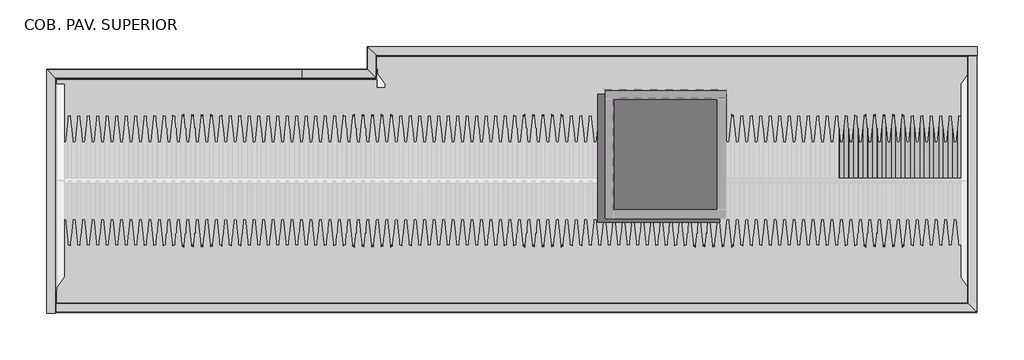
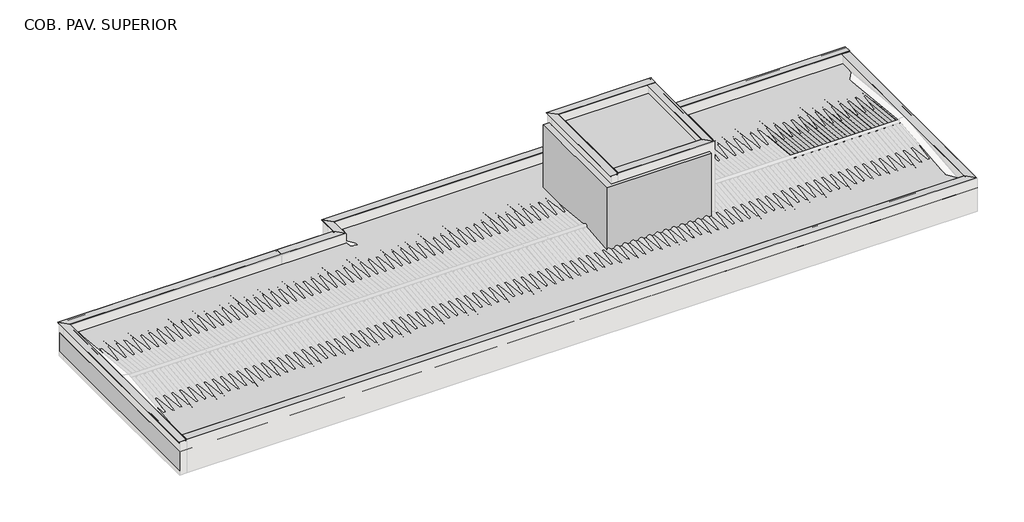
# One storey, part 8 of 8: 25 beams, 7 columns, 4 proxies.
"""IFC4 building model written with IfcOpenShell, lengths in millimetres."""

import ifcopenshell
import ifcopenshell.guid

model = None  # the IFC model being written
_history = None  # IfcOwnerHistory: only IFC2X3 demands one
_inside = {}  # id of a spatial element -> (the spatial element, [elements in it])
_under = {}  # id of a project, library or spatial element -> (it, [spatial elements below it])
_declared = {}  # id of a project -> (the project, [libraries it declares])
_typed = {}  # id of a type object -> (the type object, [elements of that type])
_made_of = {}  # id of a material, layer set ... -> (it, [elements and type objects made of it])


def new_model(schema):
    """Start an empty IFC model of exactly this schema.

    Asked for "IFC4X3", IfcOpenShell would pick the latest addendum, in which some entities
    have other attributes; the version numbers below select the first issue.
    IFC2X3 requires an IfcOwnerHistory on every rooted entity: one is made here for all.
    """
    global model, _history
    if schema == "IFC4X3":
        model = ifcopenshell.file(schema_version=(4, 3, 0, 0))
    else:
        model = ifcopenshell.file(schema=schema)
    _inside.clear()
    _under.clear()
    _declared.clear()
    _typed.clear()
    _made_of.clear()
    _history = None
    if model.schema == "IFC2X3":
        org = make("IfcOrganization", Name="unknown")
        user = make(
            "IfcPersonAndOrganization",
            ThePerson=make("IfcPerson", FamilyName="unknown"),
            TheOrganization=org,
        )
        app = make(
            "IfcApplication",
            ApplicationDeveloper=org,
            Version="unknown",
            ApplicationFullName="unknown",
            ApplicationIdentifier="unknown",
        )
        _history = make(
            "IfcOwnerHistory",
            OwningUser=user,
            OwningApplication=app,
            ChangeAction="ADDED",
            CreationDate=0,
        )
    return model


def make(cls, **values):
    """One entity of the class cls with the attributes given. An attribute that is None is left unset."""
    return model.create_entity(
        cls, **{name: value for name, value in values.items() if value is not None}
    )


def rooted(cls, **values):
    """An entity with a GlobalId (a new one), such as an element, a storey or a relation."""
    return make(cls, GlobalId=ifcopenshell.guid.new(), OwnerHistory=_history, **values)


def si_unit(unit_type, name, prefix=None):
    """IfcSIUnit, for example si_unit("LENGTHUNIT", "METRE", prefix="MILLI")."""
    return make("IfcSIUnit", UnitType=unit_type, Prefix=prefix, Name=name)


def assignment(units):
    """IfcUnitAssignment: the units of a project."""
    return None if units is None else make("IfcUnitAssignment", Units=units)


def point(xyz):
    """IfcCartesianPoint."""
    return None if xyz is None else make("IfcCartesianPoint", Coordinates=xyz)


def direction(xyz):
    """IfcDirection."""
    return None if xyz is None else make("IfcDirection", DirectionRatios=xyz)


def frame(location, z_axis=None, x_axis=None):
    """IfcAxis2Placement3D, a coordinate frame: its origin and axes. An axis left out is left unset."""
    return make(
        "IfcAxis2Placement3D",
        Location=point(location),
        Axis=direction(z_axis),
        RefDirection=direction(x_axis),
    )


def frame_2d(location, x_axis=None):
    """IfcAxis2Placement2D, a coordinate frame in the plane: its origin and x axis."""
    return make(
        "IfcAxis2Placement2D", Location=point(location), RefDirection=direction(x_axis)
    )


def origin():
    """The frame at (0, 0, 0) with its axes left unset."""
    return frame((0.0, 0.0, 0.0))


def place(relative_to, where):
    """IfcLocalPlacement: puts the frame where relative to a parent placement (None: the world)."""
    return make(
        "IfcLocalPlacement", PlacementRelTo=relative_to, RelativePlacement=where
    )


def context(
    kind, dimensions, precision=None, world=None, true_north=None, identifier=None
):
    """IfcGeometricRepresentationContext, for example the 3D "Model" context."""
    return make(
        "IfcGeometricRepresentationContext",
        ContextIdentifier=identifier,
        ContextType=kind,
        CoordinateSpaceDimension=dimensions,
        Precision=precision,
        WorldCoordinateSystem=world,
        TrueNorth=true_north,
    )


def project(units=None, contexts=None):
    """IfcProject with its units and contexts."""
    return rooted(
        "IfcProject",
        Name="project",
        RepresentationContexts=contexts,
        UnitsInContext=assignment(units),
    )


def spatial(cls, under=None, at=None, **own):
    """A site, building, storey or space (cls), placed at a placement, below another one or the project."""
    s = rooted(cls, ObjectPlacement=at, **own)
    if under is not None:
        _under.setdefault(under.id(), (under, []))[1].append(s)
    return s


def polyline(points):
    """IfcPolyline through the points."""
    return make("IfcPolyline", Points=[point(p) for p in points])


def circle_curve(where, radius):
    """IfcCircle in the frame where."""
    return make("IfcCircle", Position=where, Radius=radius)


def trimmed(basis, trim1, trim2, sense, master):
    """IfcTrimmedCurve: the piece of a basis curve between two trims."""
    return make(
        "IfcTrimmedCurve",
        BasisCurve=basis,
        Trim1=trim1,
        Trim2=trim2,
        SenseAgreement=sense,
        MasterRepresentation=master,
    )


def segment(curve, same_sense, transition):
    """IfcCompositeCurveSegment."""
    return make(
        "IfcCompositeCurveSegment",
        Transition=transition,
        SameSense=same_sense,
        ParentCurve=curve,
    )


def composite_curve(segments, self_intersect=None):
    """IfcCompositeCurve: segments joined end to end."""
    return make("IfcCompositeCurve", Segments=segments, SelfIntersect=self_intersect)


def outline(outer, holes=None, kind="AREA"):
    """IfcArbitraryClosedProfileDef: a profile drawn as a closed curve; with holes, ...WithVoids."""
    if holes is None:
        return make("IfcArbitraryClosedProfileDef", ProfileType=kind, OuterCurve=outer)
    return make(
        "IfcArbitraryProfileDefWithVoids",
        ProfileType=kind,
        OuterCurve=outer,
        InnerCurves=holes,
    )


def extrude(swept, where, along, depth):
    """IfcExtrudedAreaSolid: the profile swept, set in the frame where, extruded along a direction by depth."""
    return make(
        "IfcExtrudedAreaSolid",
        SweptArea=swept,
        Position=where,
        ExtrudedDirection=direction(along),
        Depth=depth,
    )


def faces_of(points, faces, orient=None, outer=None):
    """IfcFace entities. A face is a list of loops; a loop is a list of indices into points, from 0.

    orient and outer hold one flag for each loop. By default every Orientation is true, the
    first loop of a face is its IfcFaceOuterBound and the others are IfcFaceBound.
    """
    made = []
    for i, loops in enumerate(faces):
        bounds = []
        for j, loop in enumerate(loops):
            is_outer = j == 0 if outer is None else outer[i][j]
            bounds.append(
                make(
                    "IfcFaceOuterBound" if is_outer else "IfcFaceBound",
                    Bound=make("IfcPolyLoop", Polygon=[points[k] for k in loop]),
                    Orientation=True if orient is None else orient[i][j],
                )
            )
        made.append(make("IfcFace", Bounds=bounds))
    return made


def faceted_brep(points, faces, orient=None, outer=None, voids=None):
    """IfcFacetedBrep: a solid bounded by flat faces; with voids (closed shells), ...WithVoids."""
    shared = [point(p) for p in points]
    hull = make("IfcClosedShell", CfsFaces=faces_of(shared, faces, orient, outer))
    if voids is None:
        return make("IfcFacetedBrep", Outer=hull)
    return make(
        "IfcFacetedBrepWithVoids",
        Outer=hull,
        Voids=[
            make(cls, CfsFaces=faces_of(shared, fs, o, b)) for cls, fs, o, b in voids
        ],
    )


def shape(context_of_items, identifier, shape_type, items):
    """IfcShapeRepresentation: the items that make up one representation, for example the "Body"."""
    return make(
        "IfcShapeRepresentation",
        ContextOfItems=context_of_items,
        RepresentationIdentifier=identifier,
        RepresentationType=shape_type,
        Items=items,
    )


def source(mapping_origin, context_of_items, identifier, shape_type, items):
    """IfcRepresentationMap: a shape defined once, which mapped items show again and again."""
    return make(
        "IfcRepresentationMap",
        MappingOrigin=mapping_origin,
        MappedRepresentation=shape(context_of_items, identifier, shape_type, items),
    )


def transform(
    local_origin,
    x_axis=None,
    y_axis=None,
    z_axis=None,
    scale=None,
    scale2=None,
    scale3=None,
    uniform=True,
):
    """IfcCartesianTransformationOperator3D, or its non-uniform kind. x_axis, y_axis, z_axis: its Axis1, 2, 3."""
    if uniform:
        return make(
            "IfcCartesianTransformationOperator3D",
            Axis1=direction(x_axis),
            Axis2=direction(y_axis),
            LocalOrigin=point(local_origin),
            Scale=scale,
            Axis3=direction(z_axis),
        )
    return make(
        "IfcCartesianTransformationOperator3DnonUniform",
        Axis1=direction(x_axis),
        Axis2=direction(y_axis),
        LocalOrigin=point(local_origin),
        Scale=scale,
        Axis3=direction(z_axis),
        Scale2=scale2,
        Scale3=scale3,
    )


def mapped(mapping_source, mapping_target):
    """IfcMappedItem: shows the shape of a source again, moved by a transform."""
    return make(
        "IfcMappedItem", MappingSource=mapping_source, MappingTarget=mapping_target
    )


def made_of(thing, what):
    """Note that an element or type object is made of a material, layer set ...; save() writes the relation."""
    if what is not None:
        _made_of.setdefault(what.id(), (what, []))[1].append(thing)
    return thing


def element(
    cls,
    number,
    at=None,
    inside=None,
    cuts=None,
    type_object=None,
    material=None,
    context=None,
    identifier="Body",
    shape_type=None,
    held_by="IfcProductDefinitionShape",
    body=None,
    shapes=None,
    **own,
):
    """One element of the class cls, such as IfcWall. Its Tag is "e" and its number.

    at: its placement. inside: the storey or other place that contains it. cuts: it is an
    opening in that element (IfcRelVoidsElement). A single representation is given by context,
    identifier, shape_type and body (its items); several are given by shapes. held_by: the class
    of the entity that holds the representations. save() writes the other relations.
    """
    e = rooted(cls, Tag="e%d" % number, ObjectPlacement=at, **own)
    if body is not None:
        shapes = [shape(context, identifier, shape_type, body)]
    if shapes is not None:
        e.Representation = make(held_by, Representations=shapes)
    if inside is not None:
        _inside.setdefault(inside.id(), (inside, []))[1].append(e)
    if cuts is not None:
        rooted(
            "IfcRelVoidsElement", RelatingBuildingElement=cuts, RelatedOpeningElement=e
        )
    if type_object is not None:
        _typed.setdefault(type_object.id(), (type_object, []))[1].append(e)
    return made_of(e, material)


def aggregate(whole, parts):
    """IfcRelAggregates: a whole, such as a stair, and the parts it consists of."""
    return rooted("IfcRelAggregates", RelatingObject=whole, RelatedObjects=parts)


def save(model, path):
    """Write the relations noted so far, then the file.

    IfcRelAggregates (storeys below a building ...), IfcRelContainedInSpatialStructure (elements
    in a storey), IfcRelDefinesByType, IfcRelAssociatesMaterial and IfcRelDeclares: one each for
    every whole, place, type object, material and project.
    """
    for whole, parts in _under.values():
        aggregate(whole, parts)
    for where, things in _inside.values():
        rooted(
            "IfcRelContainedInSpatialStructure",
            RelatedElements=things,
            RelatingStructure=where,
        )
    for kind, things in _typed.values():
        rooted("IfcRelDefinesByType", RelatedObjects=things, RelatingType=kind)
    for what, things in _made_of.values():
        rooted("IfcRelAssociatesMaterial", RelatedObjects=things, RelatingMaterial=what)
    for by, libraries in _declared.values():
        rooted("IfcRelDeclares", RelatingContext=by, RelatedDefinitions=libraries)
    model.write(path)


def beam_fe4ddbad(model_context):
    return source(origin(), model_context, "Body", "SweptSolid", [
        extrude(outline(polyline([(998.8971968, 30.0), (998.8971968, -30.0), (-998.8971974, -30.0), (-998.8971974, 30.0), (998.8971968, 30.0)])), frame((0.0, 0.0, -60.0), z_axis=(0.0, 0.0, 1.0), x_axis=(1.0, 0.0, 0.0)), (0.0, 0.0, 1.0), 120.0),
    ])


def beam_88f0ebe1(model_context):
    return source(origin(), model_context, "Body", "SweptSolid", [
        extrude(outline(polyline([(136.7503096, 30.0), (136.7503096, -30.0), (-136.7503096, -30.0), (-136.7503096, 30.0), (136.7503096, 30.0)])), frame((0.0, 0.0, -60.0), z_axis=(0.0, 0.0, 1.0), x_axis=(1.0, 0.0, 0.0)), (0.0, 0.0, 1.0), 120.0),
    ])


def beam_c6e4bd39(model_context):
    return source(origin(), model_context, "Body", "SweptSolid", [
        extrude(outline(polyline([(789.5373463, 30.0), (789.5373463, -30.0), (-789.5373463, -30.0), (-789.5373463, 30.0), (789.5373463, 30.0)])), frame((0.0, 0.0, -60.0), z_axis=(0.0, 0.0, 1.0), x_axis=(1.0, 0.0, 0.0)), (0.0, 0.0, 1.0), 120.0),
    ])


def telha_ondulada_fibrocimento_963230a9(model_context):
    return source(origin(), model_context, "Body", "SweptSolid", [
        extrude(outline(composite_curve([segment(trimmed(circle_curve(frame_2d((68.3970135, 71.7939461)), 66.7939461), [point((8.3970135, 42.4437972))], [point((128.3970135, 42.4437972))], True, "CARTESIAN"), True, "CONTINUOUS"), segment(polyline([(128.3970135, 42.4437972), (132.8884385, 40.2467307)]), True, "CONTINUOUS"), segment(trimmed(circle_curve(frame_2d((68.3970135, 71.7939461)), 71.7939461), [point((132.8884385, 40.2467307))], [point((3.9055884, 40.2467307))], False, "CARTESIAN"), True, "CONTINUOUS"), segment(trimmed(circle_curve(frame_2d((-51.6029865, 13.0936483)), 61.7939461), [point((3.9055884, 40.2467307))], [point((-107.1115615, 40.2467307))], True, "CARTESIAN"), True, "CONTINUOUS"), segment(polyline([(-107.1115615, 40.2467307), (-111.6029865, 42.4437972)]), True, "CONTINUOUS"), segment(trimmed(circle_curve(frame_2d((-51.6029865, 13.0936483)), 66.7939461), [point((-111.6029865, 42.4437972))], [point((8.3970135, 42.4437972))], False, "CARTESIAN"), True, "CONTINUOUS")], self_intersect=False)), frame((-362.9289365, 0.0, 0.0), z_axis=(1.0, 0.0, 0.0), x_axis=(0.0, 1.0, 0.0)), (0.0, 0.0, 1.0), 725.8578731),
    ])


def column_6c15bf79(model_context):
    return source(origin(), model_context, "Body", "SweptSolid", [
        extrude(outline(polyline([(30.0, 80.0), (30.0, -80.0), (-30.0, -80.0), (-30.0, 80.0), (30.0, 80.0)])), frame((0.0, 0.0, 6710.0), z_axis=(0.0, 0.0, 1.0), x_axis=(1.0, 0.0, 0.0)), (0.0, 0.0, 1.0), 467.5),
    ])


def column_910cb117(model_context):
    return source(origin(), model_context, "Body", "SweptSolid", [
        extrude(outline(polyline([(30.0, 80.0), (30.0, -80.0), (-30.0, -80.0), (-30.0, 80.0), (30.0, 80.0)])), frame((0.0, 0.0, 6710.0), z_axis=(0.0, 0.0, 1.0), x_axis=(1.0, 0.0, 0.0)), (0.0, 0.0, 1.0), 371.3),
    ])


def column_42eef9f8(model_context):
    return source(origin(), model_context, "Body", "SweptSolid", [
        extrude(outline(polyline([(30.0, 80.0), (30.0, -80.0), (-30.0, -80.0), (-30.0, 80.0), (30.0, 80.0)])), frame((0.0, 0.0, 6710.0), z_axis=(0.0, 0.0, 1.0), x_axis=(1.0, 0.0, 0.0)), (0.0, 0.0, 1.0), 227.1),
    ])


model = new_model("IFC4")

# Units and contexts
model_context = context("Model", 3, world=origin())
ifc_project = project(units=[si_unit("LENGTHUNIT", "METRE", prefix="MILLI")], contexts=[model_context])

# Site, building, storey
site = spatial("IfcSite", under=ifc_project)
building = spatial("IfcBuilding", under=site)
storey = spatial("IfcBuildingStorey", under=building, Name="COB. PAV. SUPERIOR", Elevation=6650.0)

# Beams
placement = place(None, origin())
beam_shape = beam_fe4ddbad(model_context)
element("IfcBeam", 1, ObjectType="Madeira de lei : Berço 6x12cm", at=placement, inside=storey, context=model_context, shape_type="MappedRepresentation", body=[
    mapped(beam_shape, transform((9545.2046801, -7777.6209418, 6680.0), x_axis=(1.0, 0.0, 0.0), y_axis=(0.0, 0.0, -1.0), z_axis=(0.0, 1.0, 0.0))),
])
element("IfcBeam", 2, ObjectType="Madeira de lei : Berço 6x12cm", at=placement, inside=storey, context=model_context, shape_type="MappedRepresentation", body=[
    mapped(beam_shape, transform((7547.4102853, -6365.3711004, 6680.0), x_axis=(1.0, 0.0, 0.0), y_axis=(0.0, 0.0, -1.0), z_axis=(0.0, 1.0, 0.0))),
])
element("IfcBeam", 3, ObjectType="Madeira de lei : Berço 6x12cm", at=placement, inside=storey, context=model_context, shape_type="MappedRepresentation", body=[
    mapped(beam_shape, transform((9545.2046801, -6365.3711004, 6680.0), x_axis=(1.0, 0.0, 0.0), y_axis=(0.0, 0.0, -1.0), z_axis=(0.0, 1.0, 0.0))),
])
element("IfcBeam", 4, ObjectType="Madeira de lei : Berço 6x12cm", at=placement, inside=storey, context=model_context, shape_type="MappedRepresentation", body=[
    mapped(beam_shape, transform((8239.7598386, -4923.3211004, 6680.0), x_axis=(1.0, 0.0, 0.0), y_axis=(0.0, 0.0, -1.0), z_axis=(0.0, 1.0, 0.0))),
])
element("IfcBeam", 5, ObjectType="Madeira de lei : Berço 6x12cm", at=placement, inside=storey, context=model_context, shape_type="MappedRepresentation", body=[
    mapped(beam_shape, transform((6241.9654444, -4923.3211004, 6680.0), x_axis=(1.0, 0.0, 0.0), y_axis=(0.0, 0.0, -1.0), z_axis=(0.0, 1.0, 0.0))),
])
element("IfcBeam", 6, ObjectType="Madeira de lei : Berço 6x12cm", at=placement, inside=storey, context=model_context, shape_type="MappedRepresentation", body=[
    mapped(beam_shape, transform((4244.1710499, -4923.3211004, 6680.0), x_axis=(1.0, 0.0, 0.0), y_axis=(0.0, 0.0, -1.0), z_axis=(0.0, 1.0, 0.0))),
])
beam_2_shape = beam_88f0ebe1(model_context)
element("IfcBeam", 7, ObjectType="Madeira de lei : Berço 6x12cm", at=placement, inside=storey, context=model_context, shape_type="MappedRepresentation", body=[
    mapped(beam_2_shape, transform((10680.8521871, -7777.6209418, 6680.0), x_axis=(1.0, 0.0, 0.0), y_axis=(0.0, 0.0, -1.0), z_axis=(0.0, 1.0, 0.0))),
])
element("IfcBeam", 8, ObjectType="Madeira de lei : Berço 6x12cm", at=placement, inside=storey, context=model_context, shape_type="MappedRepresentation", body=[
    mapped(beam_2_shape, transform((10680.8521871, -6365.3711004, 6680.0), x_axis=(1.0, 0.0, 0.0), y_axis=(0.0, 0.0, -1.0), z_axis=(0.0, 1.0, 0.0))),
])
beam_3_shape = beam_c6e4bd39(model_context)
element("IfcBeam", 9, ObjectType="Madeira de lei : Berço 6x12cm", at=placement, inside=storey, context=model_context, shape_type="MappedRepresentation", body=[
    mapped(beam_3_shape, transform((10028.1943824, -4923.3211004, 6680.0), x_axis=(1.0, 0.0, 0.0), y_axis=(0.0, 0.0, -1.0), z_axis=(0.0, 1.0, 0.0))),
])
element("IfcBeam", 10, ObjectType="Telha Ondulada : Fibrocimento", at=placement, inside=storey, context=model_context, shape_type="SweptSolid", body=[
    extrude(outline(composite_curve([segment(trimmed(circle_curve(frame_2d((-58.7002978, -53.2060539)), 66.7939461), [point((-29.3501489, 6.7939461))], [point((-29.3501489, -113.2060539))], False, "CARTESIAN"), True, "CONTINUOUS"), segment(polyline([(-29.3501489, -113.2060539), (-31.5472154, -108.7146289)]), True, "CONTINUOUS"), segment(trimmed(circle_curve(frame_2d((-58.7002978, -53.2060539)), 61.7939461), [point((-31.5472154, -108.7146289))], [point((-31.5472154, 2.3025211))], True, "CARTESIAN"), True, "CONTINUOUS"), segment(trimmed(circle_curve(frame_2d((0.0, 66.7939461)), 71.7939461), [point((-31.5472154, 2.3025211))], [point((-31.5472154, 131.2853711))], False, "CARTESIAN"), True, "CONTINUOUS"), segment(polyline([(-31.5472154, 131.2853711), (-29.3501489, 126.7939461)]), True, "CONTINUOUS"), segment(trimmed(circle_curve(frame_2d((0.0, 66.7939461)), 66.7939461), [point((-29.3501489, 126.7939461))], [point((-29.3501489, 6.7939461))], True, "CARTESIAN"), True, "CONTINUOUS")], self_intersect=False)), frame((7596.2156257, -4723.1805671, 7106.8215886), z_axis=(0.0, -0.9950371902099893, 0.09950371902099783), x_axis=(0.0, 0.09950371902099783, 0.9950371902099893)), (0.0, 0.0, 1.0), 3060.4439799),
])
element("IfcBeam", 11, ObjectType="Telha Ondulada : Fibrocimento", at=placement, inside=storey, context=model_context, shape_type="SweptSolid", body=[
    extrude(outline(composite_curve([segment(trimmed(circle_curve(frame_2d((-58.7002978, -53.2060539)), 66.7939461), [point((-29.3501489, 6.7939461))], [point((-29.3501489, -113.2060539))], False, "CARTESIAN"), True, "CONTINUOUS"), segment(polyline([(-29.3501489, -113.2060539), (-31.5472154, -108.7146289)]), True, "CONTINUOUS"), segment(trimmed(circle_curve(frame_2d((-58.7002978, -53.2060539)), 61.7939461), [point((-31.5472154, -108.7146289))], [point((-31.5472154, 2.3025211))], True, "CARTESIAN"), True, "CONTINUOUS"), segment(trimmed(circle_curve(frame_2d((0.0, 66.7939461)), 71.7939461), [point((-31.5472154, 2.3025211))], [point((-31.5472154, 131.2853711))], False, "CARTESIAN"), True, "CONTINUOUS"), segment(polyline([(-31.5472154, 131.2853711), (-29.3501489, 126.7939461)]), True, "CONTINUOUS"), segment(trimmed(circle_curve(frame_2d((0.0, 66.7939461)), 66.7939461), [point((-29.3501489, 126.7939461))], [point((-29.3501489, 6.7939461))], True, "CARTESIAN"), True, "CONTINUOUS")], self_intersect=False)), frame((7840.7156257, -4723.1805671, 7106.8215886), z_axis=(0.0, -0.9950371902099893, 0.09950371902099783), x_axis=(0.0, 0.09950371902099783, 0.9950371902099893)), (0.0, 0.0, 1.0), 3060.4439799),
])
element("IfcBeam", 12, ObjectType="Telha Ondulada : Fibrocimento", at=placement, inside=storey, context=model_context, shape_type="SweptSolid", body=[
    extrude(outline(composite_curve([segment(trimmed(circle_curve(frame_2d((-58.7002978, -53.2060539)), 66.7939461), [point((-29.3501489, 6.7939461))], [point((-29.3501489, -113.2060539))], False, "CARTESIAN"), True, "CONTINUOUS"), segment(polyline([(-29.3501489, -113.2060539), (-31.5472154, -108.7146289)]), True, "CONTINUOUS"), segment(trimmed(circle_curve(frame_2d((-58.7002978, -53.2060539)), 61.7939461), [point((-31.5472154, -108.7146289))], [point((-31.5472154, 2.3025211))], True, "CARTESIAN"), True, "CONTINUOUS"), segment(trimmed(circle_curve(frame_2d((0.0, 66.7939461)), 71.7939461), [point((-31.5472154, 2.3025211))], [point((-31.5472154, 131.2853711))], False, "CARTESIAN"), True, "CONTINUOUS"), segment(polyline([(-31.5472154, 131.2853711), (-29.3501489, 126.7939461)]), True, "CONTINUOUS"), segment(trimmed(circle_curve(frame_2d((0.0, 66.7939461)), 66.7939461), [point((-29.3501489, 126.7939461))], [point((-29.3501489, 6.7939461))], True, "CARTESIAN"), True, "CONTINUOUS")], self_intersect=False)), frame((8085.2156257, -4723.1805671, 7106.8215886), z_axis=(0.0, -0.9950371902099893, 0.09950371902099783), x_axis=(0.0, 0.09950371902099783, 0.9950371902099893)), (0.0, 0.0, 1.0), 3060.4439799),
])
element("IfcBeam", 13, ObjectType="Telha Ondulada : Fibrocimento", at=placement, inside=storey, context=model_context, shape_type="SweptSolid", body=[
    extrude(outline(composite_curve([segment(trimmed(circle_curve(frame_2d((-58.7002978, -53.2060539)), 66.7939461), [point((-29.3501489, 6.7939461))], [point((-29.3501489, -113.2060539))], False, "CARTESIAN"), True, "CONTINUOUS"), segment(polyline([(-29.3501489, -113.2060539), (-31.5472154, -108.7146289)]), True, "CONTINUOUS"), segment(trimmed(circle_curve(frame_2d((-58.7002978, -53.2060539)), 61.7939461), [point((-31.5472154, -108.7146289))], [point((-31.5472154, 2.3025211))], True, "CARTESIAN"), True, "CONTINUOUS"), segment(trimmed(circle_curve(frame_2d((0.0, 66.7939461)), 71.7939461), [point((-31.5472154, 2.3025211))], [point((-31.5472154, 131.2853711))], False, "CARTESIAN"), True, "CONTINUOUS"), segment(polyline([(-31.5472154, 131.2853711), (-29.3501489, 126.7939461)]), True, "CONTINUOUS"), segment(trimmed(circle_curve(frame_2d((0.0, 66.7939461)), 66.7939461), [point((-29.3501489, 126.7939461))], [point((-29.3501489, 6.7939461))], True, "CARTESIAN"), True, "CONTINUOUS")], self_intersect=False)), frame((8329.7156257, -4723.1805671, 7106.8215886), z_axis=(0.0, -0.9950371902099893, 0.09950371902099785), x_axis=(0.0, 0.09950371902099785, 0.9950371902099893)), (0.0, 0.0, 1.0), 3060.4439799),
])
element("IfcBeam", 14, ObjectType="Telha Ondulada : Fibrocimento", at=placement, inside=storey, context=model_context, shape_type="SweptSolid", body=[
    extrude(outline(composite_curve([segment(trimmed(circle_curve(frame_2d((-58.7002978, -53.2060539)), 66.7939461), [point((-29.3501489, 6.7939461))], [point((-29.3501489, -113.2060539))], False, "CARTESIAN"), True, "CONTINUOUS"), segment(polyline([(-29.3501489, -113.2060539), (-31.5472154, -108.7146289)]), True, "CONTINUOUS"), segment(trimmed(circle_curve(frame_2d((-58.7002978, -53.2060539)), 61.7939461), [point((-31.5472154, -108.7146289))], [point((-31.5472154, 2.3025211))], True, "CARTESIAN"), True, "CONTINUOUS"), segment(trimmed(circle_curve(frame_2d((0.0, 66.7939461)), 71.7939461), [point((-31.5472154, 2.3025211))], [point((-31.5472154, 131.2853711))], False, "CARTESIAN"), True, "CONTINUOUS"), segment(polyline([(-31.5472154, 131.2853711), (-29.3501489, 126.7939461)]), True, "CONTINUOUS"), segment(trimmed(circle_curve(frame_2d((0.0, 66.7939461)), 66.7939461), [point((-29.3501489, 126.7939461))], [point((-29.3501489, 6.7939461))], True, "CARTESIAN"), True, "CONTINUOUS")], self_intersect=False)), frame((8574.2156257, -4723.1805671, 7106.8215886), z_axis=(0.0, -0.9950371902099893, 0.0995037190209978), x_axis=(0.0, 0.0995037190209978, 0.9950371902099893)), (0.0, 0.0, 1.0), 3060.4439799),
])
element("IfcBeam", 15, ObjectType="Telha Ondulada : Fibrocimento", at=placement, inside=storey, context=model_context, shape_type="SweptSolid", body=[
    extrude(outline(composite_curve([segment(trimmed(circle_curve(frame_2d((-58.7002978, -53.2060539)), 66.7939461), [point((-29.3501489, 6.7939461))], [point((-29.3501489, -113.2060539))], False, "CARTESIAN"), True, "CONTINUOUS"), segment(polyline([(-29.3501489, -113.2060539), (-31.5472154, -108.7146289)]), True, "CONTINUOUS"), segment(trimmed(circle_curve(frame_2d((-58.7002978, -53.2060539)), 61.7939461), [point((-31.5472154, -108.7146289))], [point((-31.5472154, 2.3025211))], True, "CARTESIAN"), True, "CONTINUOUS"), segment(trimmed(circle_curve(frame_2d((0.0, 66.7939461)), 71.7939461), [point((-31.5472154, 2.3025211))], [point((-31.5472154, 131.2853711))], False, "CARTESIAN"), True, "CONTINUOUS"), segment(polyline([(-31.5472154, 131.2853711), (-29.3501489, 126.7939461)]), True, "CONTINUOUS"), segment(trimmed(circle_curve(frame_2d((0.0, 66.7939461)), 66.7939461), [point((-29.3501489, 126.7939461))], [point((-29.3501489, 6.7939461))], True, "CARTESIAN"), True, "CONTINUOUS")], self_intersect=False)), frame((8818.7156257, -4723.1805671, 7106.8215886), z_axis=(0.0, -0.9950371902099893, 0.0995037190209978), x_axis=(0.0, 0.0995037190209978, 0.9950371902099893)), (0.0, 0.0, 1.0), 3060.4439799),
])
element("IfcBeam", 16, ObjectType="Telha Ondulada : Fibrocimento", at=placement, inside=storey, context=model_context, shape_type="SweptSolid", body=[
    extrude(outline(composite_curve([segment(trimmed(circle_curve(frame_2d((-58.7002978, -53.2060539)), 66.7939461), [point((-29.3501489, 6.7939461))], [point((-29.3501489, -113.2060539))], False, "CARTESIAN"), True, "CONTINUOUS"), segment(polyline([(-29.3501489, -113.2060539), (-31.5472154, -108.7146289)]), True, "CONTINUOUS"), segment(trimmed(circle_curve(frame_2d((-58.7002978, -53.2060539)), 61.7939461), [point((-31.5472154, -108.7146289))], [point((-31.5472154, 2.3025211))], True, "CARTESIAN"), True, "CONTINUOUS"), segment(trimmed(circle_curve(frame_2d((0.0, 66.7939461)), 71.7939461), [point((-31.5472154, 2.3025211))], [point((-31.5472154, 131.2853711))], False, "CARTESIAN"), True, "CONTINUOUS"), segment(polyline([(-31.5472154, 131.2853711), (-29.3501489, 126.7939461)]), True, "CONTINUOUS"), segment(trimmed(circle_curve(frame_2d((0.0, 66.7939461)), 66.7939461), [point((-29.3501489, 126.7939461))], [point((-29.3501489, 6.7939461))], True, "CARTESIAN"), True, "CONTINUOUS")], self_intersect=False)), frame((9063.2156257, -4723.1805671, 7106.8215886), z_axis=(0.0, -0.9950371902099893, 0.0995037190209978), x_axis=(0.0, 0.0995037190209978, 0.9950371902099893)), (0.0, 0.0, 1.0), 3060.4439799),
])
element("IfcBeam", 17, ObjectType="Telha Ondulada : Fibrocimento", at=placement, inside=storey, context=model_context, shape_type="SweptSolid", body=[
    extrude(outline(composite_curve([segment(trimmed(circle_curve(frame_2d((-58.7002978, -53.2060539)), 66.7939461), [point((-29.3501489, 6.7939461))], [point((-29.3501489, -113.2060539))], False, "CARTESIAN"), True, "CONTINUOUS"), segment(polyline([(-29.3501489, -113.2060539), (-31.5472154, -108.7146289)]), True, "CONTINUOUS"), segment(trimmed(circle_curve(frame_2d((-58.7002978, -53.2060539)), 61.7939461), [point((-31.5472154, -108.7146289))], [point((-31.5472154, 2.3025211))], True, "CARTESIAN"), True, "CONTINUOUS"), segment(trimmed(circle_curve(frame_2d((0.0, 66.7939461)), 71.7939461), [point((-31.5472154, 2.3025211))], [point((-31.5472154, 131.2853711))], False, "CARTESIAN"), True, "CONTINUOUS"), segment(polyline([(-31.5472154, 131.2853711), (-29.3501489, 126.7939461)]), True, "CONTINUOUS"), segment(trimmed(circle_curve(frame_2d((0.0, 66.7939461)), 66.7939461), [point((-29.3501489, 126.7939461))], [point((-29.3501489, 6.7939461))], True, "CARTESIAN"), True, "CONTINUOUS")], self_intersect=False)), frame((9307.7156257, -4723.1805671, 7106.8215886), z_axis=(0.0, -0.9950371902099893, 0.0995037190209978), x_axis=(0.0, 0.0995037190209978, 0.9950371902099893)), (0.0, 0.0, 1.0), 3060.4439799),
])
element("IfcBeam", 18, ObjectType="Telha Ondulada : Fibrocimento", at=placement, inside=storey, context=model_context, shape_type="SweptSolid", body=[
    extrude(outline(composite_curve([segment(trimmed(circle_curve(frame_2d((-58.7002978, -53.2060539)), 66.7939461), [point((-29.3501489, 6.7939461))], [point((-29.3501489, -113.2060539))], False, "CARTESIAN"), True, "CONTINUOUS"), segment(polyline([(-29.3501489, -113.2060539), (-31.5472154, -108.7146289)]), True, "CONTINUOUS"), segment(trimmed(circle_curve(frame_2d((-58.7002978, -53.2060539)), 61.7939461), [point((-31.5472154, -108.7146289))], [point((-31.5472154, 2.3025211))], True, "CARTESIAN"), True, "CONTINUOUS"), segment(trimmed(circle_curve(frame_2d((0.0, 66.7939461)), 71.7939461), [point((-31.5472154, 2.3025211))], [point((-31.5472154, 131.2853711))], False, "CARTESIAN"), True, "CONTINUOUS"), segment(polyline([(-31.5472154, 131.2853711), (-29.3501489, 126.7939461)]), True, "CONTINUOUS"), segment(trimmed(circle_curve(frame_2d((0.0, 66.7939461)), 66.7939461), [point((-29.3501489, 126.7939461))], [point((-29.3501489, 6.7939461))], True, "CARTESIAN"), True, "CONTINUOUS")], self_intersect=False)), frame((9552.2156257, -4723.1805671, 7106.8215886), z_axis=(0.0, -0.9950371902099893, 0.0995037190209978), x_axis=(0.0, 0.0995037190209978, 0.9950371902099893)), (0.0, 0.0, 1.0), 3060.4439799),
])
element("IfcBeam", 19, ObjectType="Telha Ondulada : Fibrocimento", at=placement, inside=storey, context=model_context, shape_type="SweptSolid", body=[
    extrude(outline(composite_curve([segment(trimmed(circle_curve(frame_2d((-58.7002978, -53.2060539)), 66.7939461), [point((-29.3501489, 6.7939461))], [point((-29.3501489, -113.2060539))], False, "CARTESIAN"), True, "CONTINUOUS"), segment(polyline([(-29.3501489, -113.2060539), (-31.5472154, -108.7146289)]), True, "CONTINUOUS"), segment(trimmed(circle_curve(frame_2d((-58.7002978, -53.2060539)), 61.7939461), [point((-31.5472154, -108.7146289))], [point((-31.5472154, 2.3025211))], True, "CARTESIAN"), True, "CONTINUOUS"), segment(trimmed(circle_curve(frame_2d((0.0, 66.7939461)), 71.7939461), [point((-31.5472154, 2.3025211))], [point((-31.5472154, 131.2853711))], False, "CARTESIAN"), True, "CONTINUOUS"), segment(polyline([(-31.5472154, 131.2853711), (-29.3501489, 126.7939461)]), True, "CONTINUOUS"), segment(trimmed(circle_curve(frame_2d((0.0, 66.7939461)), 66.7939461), [point((-29.3501489, 126.7939461))], [point((-29.3501489, 6.7939461))], True, "CARTESIAN"), True, "CONTINUOUS")], self_intersect=False)), frame((9796.7156257, -4723.1805671, 7106.8215886), z_axis=(0.0, -0.9950371902099893, 0.0995037190209978), x_axis=(0.0, 0.0995037190209978, 0.9950371902099893)), (0.0, 0.0, 1.0), 3060.4439799),
])
element("IfcBeam", 20, ObjectType="Telha Ondulada : Fibrocimento", at=placement, inside=storey, context=model_context, shape_type="SweptSolid", body=[
    extrude(outline(composite_curve([segment(trimmed(circle_curve(frame_2d((-58.7002978, -53.2060539)), 66.7939461), [point((-29.3501489, 6.7939461))], [point((-29.3501489, -113.2060539))], False, "CARTESIAN"), True, "CONTINUOUS"), segment(polyline([(-29.3501489, -113.2060539), (-31.5472154, -108.7146289)]), True, "CONTINUOUS"), segment(trimmed(circle_curve(frame_2d((-58.7002978, -53.2060539)), 61.7939461), [point((-31.5472154, -108.7146289))], [point((-31.5472154, 2.3025211))], True, "CARTESIAN"), True, "CONTINUOUS"), segment(trimmed(circle_curve(frame_2d((0.0, 66.7939461)), 71.7939461), [point((-31.5472154, 2.3025211))], [point((-31.5472154, 131.2853711))], False, "CARTESIAN"), True, "CONTINUOUS"), segment(polyline([(-31.5472154, 131.2853711), (-29.3501489, 126.7939461)]), True, "CONTINUOUS"), segment(trimmed(circle_curve(frame_2d((0.0, 66.7939461)), 66.7939461), [point((-29.3501489, 126.7939461))], [point((-29.3501489, 6.7939461))], True, "CARTESIAN"), True, "CONTINUOUS")], self_intersect=False)), frame((10041.2156257, -4723.1805671, 7106.8215886), z_axis=(0.0, -0.9950371902099893, 0.0995037190209978), x_axis=(0.0, 0.0995037190209978, 0.9950371902099893)), (0.0, 0.0, 1.0), 3060.4439799),
])
element("IfcBeam", 21, ObjectType="Telha Ondulada : Fibrocimento", at=placement, inside=storey, context=model_context, shape_type="SweptSolid", body=[
    extrude(outline(composite_curve([segment(trimmed(circle_curve(frame_2d((-58.7002978, -53.2060539)), 66.7939461), [point((-29.3501489, 6.7939461))], [point((-29.3501489, -113.2060539))], False, "CARTESIAN"), True, "CONTINUOUS"), segment(polyline([(-29.3501489, -113.2060539), (-31.5472154, -108.7146289)]), True, "CONTINUOUS"), segment(trimmed(circle_curve(frame_2d((-58.7002978, -53.2060539)), 61.7939461), [point((-31.5472154, -108.7146289))], [point((-31.5472154, 2.3025211))], True, "CARTESIAN"), True, "CONTINUOUS"), segment(trimmed(circle_curve(frame_2d((0.0, 66.7939461)), 71.7939461), [point((-31.5472154, 2.3025211))], [point((-31.5472154, 131.2853711))], False, "CARTESIAN"), True, "CONTINUOUS"), segment(polyline([(-31.5472154, 131.2853711), (-29.3501489, 126.7939461)]), True, "CONTINUOUS"), segment(trimmed(circle_curve(frame_2d((0.0, 66.7939461)), 66.7939461), [point((-29.3501489, 126.7939461))], [point((-29.3501489, 6.7939461))], True, "CARTESIAN"), True, "CONTINUOUS")], self_intersect=False)), frame((10285.7156257, -4723.1805671, 7106.8215886), z_axis=(0.0, -0.9950371902099893, 0.0995037190209978), x_axis=(0.0, 0.0995037190209978, 0.9950371902099893)), (0.0, 0.0, 1.0), 3060.4439799),
])
element("IfcBeam", 22, ObjectType="Telha Ondulada : Fibrocimento", at=placement, inside=storey, context=model_context, shape_type="SweptSolid", body=[
    extrude(outline(composite_curve([segment(trimmed(circle_curve(frame_2d((-58.7002978, -53.2060539)), 66.7939461), [point((-29.3501489, 6.7939461))], [point((-29.3501489, -113.2060539))], False, "CARTESIAN"), True, "CONTINUOUS"), segment(polyline([(-29.3501489, -113.2060539), (-31.5472154, -108.7146289)]), True, "CONTINUOUS"), segment(trimmed(circle_curve(frame_2d((-58.7002978, -53.2060539)), 61.7939461), [point((-31.5472154, -108.7146289))], [point((-31.5472154, 2.3025211))], True, "CARTESIAN"), True, "CONTINUOUS"), segment(trimmed(circle_curve(frame_2d((0.0, 66.7939461)), 71.7939461), [point((-31.5472154, 2.3025211))], [point((-31.5472154, 131.2853711))], False, "CARTESIAN"), True, "CONTINUOUS"), segment(polyline([(-31.5472154, 131.2853711), (-29.3501489, 126.7939461)]), True, "CONTINUOUS"), segment(trimmed(circle_curve(frame_2d((0.0, 66.7939461)), 66.7939461), [point((-29.3501489, 126.7939461))], [point((-29.3501489, 6.7939461))], True, "CARTESIAN"), True, "CONTINUOUS")], self_intersect=False)), frame((10530.2156257, -4723.1805671, 7106.8215886), z_axis=(0.0, -0.9950371902099893, 0.0995037190209978), x_axis=(0.0, 0.0995037190209978, 0.9950371902099893)), (0.0, 0.0, 1.0), 3060.4439799),
])
element("IfcBeam", 23, ObjectType="Telha Ondulada : Fibrocimento", at=placement, inside=storey, context=model_context, shape_type="SweptSolid", body=[
    extrude(outline(composite_curve([segment(trimmed(circle_curve(frame_2d((-58.7002978, -53.2060539)), 66.7939461), [point((-29.3501489, 6.7939461))], [point((-29.3501489, -113.2060539))], False, "CARTESIAN"), True, "CONTINUOUS"), segment(polyline([(-29.3501489, -113.2060539), (-31.5472154, -108.7146289)]), True, "CONTINUOUS"), segment(trimmed(circle_curve(frame_2d((-58.7002978, -53.2060539)), 61.7939461), [point((-31.5472154, -108.7146289))], [point((-31.5472154, 2.3025211))], True, "CARTESIAN"), True, "CONTINUOUS"), segment(trimmed(circle_curve(frame_2d((0.0, 66.7939461)), 71.7939461), [point((-31.5472154, 2.3025211))], [point((-31.5472154, 131.2853711))], False, "CARTESIAN"), True, "CONTINUOUS"), segment(polyline([(-31.5472154, 131.2853711), (-29.3501489, 126.7939461)]), True, "CONTINUOUS"), segment(trimmed(circle_curve(frame_2d((0.0, 66.7939461)), 66.7939461), [point((-29.3501489, 126.7939461))], [point((-29.3501489, 6.7939461))], True, "CARTESIAN"), True, "CONTINUOUS")], self_intersect=False)), frame((10774.7156257, -4723.1805671, 7106.8215886), z_axis=(0.0, -0.9950371902099893, 0.0995037190209978), x_axis=(0.0, 0.0995037190209978, 0.9950371902099893)), (0.0, 0.0, 1.0), 3060.4439799),
])
telha_ondulada_fibrocimento_shape = telha_ondulada_fibrocimento_963230a9(model_context)
element("IfcBeam", 24, ObjectType="Telha Ondulada : Fibrocimento", at=placement, inside=storey, context=model_context, shape_type="MappedRepresentation", body=[
    mapped(telha_ondulada_fibrocimento_shape, transform((4174.818693, -5091.4521211, 7071.4967211), x_axis=(0.0, 0.9950371902099892, -0.09950371902099847), y_axis=(-1.0, 0.0, 0.0), z_axis=(0.0, 0.09950371902099849, 0.9950371902099893))),
])
element("IfcBeam", 25, ObjectType="Telha Ondulada : Fibrocimento", at=placement, inside=storey, context=model_context, shape_type="MappedRepresentation", body=[
    mapped(telha_ondulada_fibrocimento_shape, transform((4419.318693, -5091.4521211, 7071.4967211), x_axis=(0.0, 0.9950371902099892, -0.09950371902099847), y_axis=(-1.0, 0.0, 0.0), z_axis=(0.0, 0.09950371902099849, 0.9950371902099893))),
])

# Proxies
element("IfcBuildingElementProxy", 26, Name="VOLUME DA CAIXA D'ÁGUA : VOLUME DA CAIXA D'ÁGUA", ObjectType="VOLUME DA CAIXA D'ÁGUA : VOLUME DA CAIXA D'ÁGUA", at=placement, inside=storey, context=model_context, shape_type="SweptSolid", body=[
    extrude(outline(polyline([(4389.718693, -5545.5699847), (4389.718693, -8845.5699847), (1239.718693, -8845.5699847), (1239.718693, -5545.5699847), (4389.718693, -5545.5699847)])), frame((0.0, 0.0, 6650.0), z_axis=(0.0, 0.0, 1.0), x_axis=(1.0, 0.0, 0.0)), (0.0, 0.0, 1.0), 2600.0),
])
element("IfcBuildingElementProxy", 27, Name=".CC_RUFO_PINGADEIRA_22 cm", ObjectType=".CC_RUFO_PINGADEIRA_22 cm", at=placement, inside=storey, context=model_context, shape_type="Brep", body=[
    faceted_brep([(-12737.081307, -10962.3488472, 7526.6820963), (-12737.081307, -10969.419915, 7533.7531641), (-12737.081307, -10969.419915, 7536.5815912), (-12737.081307, -10962.8458336, 7530.0075098), (-12737.081307, -10946.8985437, 7560.0), (-12737.081307, -11170.2414257, 7560.0), (-12737.081307, -11154.2941358, 7530.0075098), (-12737.081307, -11147.7200544, 7536.5815912), (-12737.081307, -11147.7200544, 7533.7531641), (-12737.081307, -11154.7911222, 7526.6820963), (-12737.081307, -11173.5699847, 7562.0), (-12737.081307, -10943.5699847, 7562.0), (10806.4975555, -10962.3488472, 7526.6820963), (10787.718693, -10943.5699847, 7562.0), (11017.718693, -11173.5699847, 7562.0), (10998.9398305, -11154.7911222, 7526.6820963), (10991.8687627, -11147.7200544, 7533.7531641), (10991.8687627, -11147.7200544, 7536.5815912), (10998.4428441, -11154.2941358, 7530.0075098), (11014.3901341, -11170.2414257, 7560.0), (10791.047252, -10946.8985437, 7560.0), (10806.9945419, -10962.8458336, 7530.0075098), (10813.5686234, -10969.419915, 7536.5815912), (10813.5686234, -10969.419915, 7533.7531641)], [[[0, 1, 2, 3, 4, 5, 6, 7, 8, 9, 10, 11]], [[12, 13, 14, 15, 16, 17, 18, 19, 20, 21, 22, 23]], [[1, 0, 12, 23]], [[2, 1, 23, 22]], [[3, 2, 22, 21]], [[4, 3, 21, 20]], [[5, 4, 20, 19]], [[6, 5, 19, 18]], [[7, 6, 18, 17]], [[8, 7, 17, 16]], [[9, 8, 16, 15]], [[10, 9, 15, 14]], [[11, 10, 14, 13]], [[0, 11, 13, 12]]]),
    faceted_brep([(-12970.3024445, -4923.3488472, 7526.6820963), (-12989.081307, -4904.5699847, 7562.0), (-12759.081307, -5134.5699847, 7562.0), (-12777.8601695, -5115.7911222, 7526.6820963), (-12784.9312373, -5108.7200544, 7533.7531641), (-12784.9312373, -5108.7200544, 7536.5815912), (-12778.3571559, -5115.2941358, 7530.0075098), (-12762.4098659, -5131.2414257, 7560.0), (-12985.752748, -4907.8985437, 7560.0), (-12969.8054581, -4923.8458336, 7530.0075098), (-12963.2313766, -4930.419915, 7536.5815912), (-12963.2313766, -4930.419915, 7533.7531641), (-12970.3024445, -11195.5699847, 7526.6820963), (-12963.2313766, -11195.5699847, 7533.7531641), (-12963.2313766, -11195.5699847, 7536.5815912), (-12969.8054581, -11195.5699847, 7530.0075098), (-12985.752748, -11195.5699847, 7560.0), (-12762.4098659, -11195.5699847, 7560.0), (-12778.3571559, -11195.5699847, 7530.0075098), (-12784.9312373, -11195.5699847, 7536.5815912), (-12784.9312373, -11195.5699847, 7533.7531641), (-12777.8601695, -11195.5699847, 7526.6820963), (-12759.081307, -11195.5699847, 7562.0), (-12989.081307, -11195.5699847, 7562.0)], [[[0, 1, 2, 3, 4, 5, 6, 7, 8, 9, 10, 11]], [[12, 13, 14, 15, 16, 17, 18, 19, 20, 21, 22, 23]], [[1, 0, 12, 23]], [[2, 1, 23, 22]], [[3, 2, 22, 21]], [[4, 3, 21, 20]], [[5, 4, 20, 19]], [[6, 5, 19, 18]], [[7, 6, 18, 17]], [[8, 7, 17, 16]], [[9, 8, 16, 15]], [[10, 9, 15, 14]], [[11, 10, 14, 13]], [[0, 11, 13, 12]]]),
    faceted_brep([(-6405.7925289, -4923.3488472, 7526.6820963), (-6405.7925289, -4904.5699847, 7562.0), (-6405.7925289, -5134.5699847, 7562.0), (-6405.7925289, -5115.7911222, 7526.6820963), (-6405.7925289, -5108.7200544, 7533.7531641), (-6405.7925289, -5108.7200544, 7536.5815912), (-6405.7925289, -5115.2941358, 7530.0075098), (-6405.7925289, -5131.2414257, 7560.0), (-6405.7925289, -4907.8985437, 7560.0), (-6405.7925289, -4923.8458336, 7530.0075098), (-6405.7925289, -4930.419915, 7536.5815912), (-6405.7925289, -4930.419915, 7533.7531641), (-12970.3024445, -4923.3488472, 7526.6820963), (-12963.2313766, -4930.419915, 7533.7531641), (-12963.2313766, -4930.419915, 7536.5815912), (-12969.8054581, -4923.8458336, 7530.0075098), (-12985.752748, -4907.8985437, 7560.0), (-12762.4098659, -5131.2414257, 7560.0), (-12778.3571559, -5115.2941358, 7530.0075098), (-12784.9312373, -5108.7200544, 7536.5815912), (-12784.9312373, -5108.7200544, 7533.7531641), (-12777.8601695, -5115.7911222, 7526.6820963), (-12759.081307, -5134.5699847, 7562.0), (-12989.081307, -4904.5699847, 7562.0)], [[[0, 1, 2, 3, 4, 5, 6, 7, 8, 9, 10, 11]], [[12, 13, 14, 15, 16, 17, 18, 19, 20, 21, 22, 23]], [[1, 0, 12, 23]], [[2, 1, 23, 22]], [[3, 2, 22, 21]], [[4, 3, 21, 20]], [[5, 4, 20, 19]], [[6, 5, 19, 18]], [[7, 6, 18, 17]], [[8, 7, 17, 16]], [[9, 8, 16, 15]], [[10, 9, 15, 14]], [[11, 10, 14, 13]], [[0, 11, 13, 12]]]),
    faceted_brep([(-4690.7187887, -4923.3488472, 7526.6820963), (-4709.4976512, -4904.5699847, 7562.0), (-4479.4976512, -5134.5699847, 7562.0), (-4498.2765137, -5115.7911222, 7526.6820963), (-4505.3475816, -5108.7200544, 7533.7531641), (-4505.3475816, -5108.7200544, 7536.5815912), (-4498.7735001, -5115.2941358, 7530.0075098), (-4482.8262102, -5131.2414257, 7560.0), (-4706.1690923, -4907.8985437, 7560.0), (-4690.2218023, -4923.8458336, 7530.0075098), (-4683.6477209, -4930.419915, 7536.5815912), (-4683.6477209, -4930.419915, 7533.7531641), (-6405.7925289, -4923.3488472, 7526.6820963), (-6405.7925289, -4930.419915, 7533.7531641), (-6405.7925289, -4930.419915, 7536.5815912), (-6405.7925289, -4923.8458336, 7530.0075098), (-6405.7925289, -4907.8985437, 7560.0), (-6405.7925289, -5131.2414257, 7560.0), (-6405.7925289, -5115.2941358, 7530.0075098), (-6405.7925289, -5108.7200544, 7536.5815912), (-6405.7925289, -5108.7200544, 7533.7531641), (-6405.7925289, -5115.7911222, 7526.6820963), (-6405.7925289, -5134.5699847, 7562.0), (-6405.7925289, -4904.5699847, 7562.0)], [[[0, 1, 2, 3, 4, 5, 6, 7, 8, 9, 10, 11]], [[12, 13, 14, 15, 16, 17, 18, 19, 20, 21, 22, 23]], [[1, 0, 12, 23]], [[2, 1, 23, 22]], [[3, 2, 22, 21]], [[4, 3, 21, 20]], [[5, 4, 20, 19]], [[6, 5, 19, 18]], [[7, 6, 18, 17]], [[8, 7, 17, 16]], [[9, 8, 16, 15]], [[10, 9, 15, 14]], [[11, 10, 14, 13]], [[0, 11, 13, 12]]]),
    faceted_brep([(-4690.7187887, -4334.3488472, 7526.6820963), (-4709.4976512, -4315.5699847, 7562.0), (-4479.4976512, -4545.5699847, 7562.0), (-4498.2765137, -4526.7911222, 7526.6820963), (-4505.3475816, -4519.7200544, 7533.7531641), (-4505.3475816, -4519.7200544, 7536.5815912), (-4498.7735001, -4526.2941358, 7530.0075098), (-4482.8262102, -4542.2414257, 7560.0), (-4706.1690923, -4318.8985437, 7560.0), (-4690.2218023, -4334.8458336, 7530.0075098), (-4683.6477209, -4341.419915, 7536.5815912), (-4683.6477209, -4341.419915, 7533.7531641), (-4690.7187887, -4923.3488472, 7526.6820963), (-4683.6477209, -4930.419915, 7533.7531641), (-4683.6477209, -4930.419915, 7536.5815912), (-4690.2218023, -4923.8458336, 7530.0075098), (-4706.1690923, -4907.8985437, 7560.0), (-4482.8262102, -5131.2414257, 7560.0), (-4498.7735001, -5115.2941358, 7530.0075098), (-4505.3475816, -5108.7200544, 7536.5815912), (-4505.3475816, -5108.7200544, 7533.7531641), (-4498.2765137, -5115.7911222, 7526.6820963), (-4479.4976512, -5134.5699847, 7562.0), (-4709.4976512, -4904.5699847, 7562.0)], [[[0, 1, 2, 3, 4, 5, 6, 7, 8, 9, 10, 11]], [[12, 13, 14, 15, 16, 17, 18, 19, 20, 21, 22, 23]], [[1, 0, 12, 23]], [[2, 1, 23, 22]], [[3, 2, 22, 21]], [[4, 3, 21, 20]], [[5, 4, 20, 19]], [[6, 5, 19, 18]], [[7, 6, 18, 17]], [[8, 7, 17, 16]], [[9, 8, 16, 15]], [[10, 9, 15, 14]], [[11, 10, 14, 13]], [[0, 11, 13, 12]]]),
    faceted_brep([(11039.718693, -4334.3488472, 7526.6820963), (11039.718693, -4315.5699847, 7562.0), (11039.718693, -4545.5699847, 7562.0), (11039.718693, -4526.7911222, 7526.6820963), (11039.718693, -4519.7200544, 7533.7531641), (11039.718693, -4519.7200544, 7536.5815912), (11039.718693, -4526.2941358, 7530.0075098), (11039.718693, -4542.2414257, 7560.0), (11039.718693, -4318.8985437, 7560.0), (11039.718693, -4334.8458336, 7530.0075098), (11039.718693, -4341.419915, 7536.5815912), (11039.718693, -4341.419915, 7533.7531641), (-4690.7187887, -4334.3488472, 7526.6820963), (-4683.6477209, -4341.419915, 7533.7531641), (-4683.6477209, -4341.419915, 7536.5815912), (-4690.2218023, -4334.8458336, 7530.0075098), (-4706.1690923, -4318.8985437, 7560.0), (-4482.8262102, -4542.2414257, 7560.0), (-4498.7735001, -4526.2941358, 7530.0075098), (-4505.3475816, -4519.7200544, 7536.5815912), (-4505.3475816, -4519.7200544, 7533.7531641), (-4498.2765137, -4526.7911222, 7526.6820963), (-4479.4976512, -4545.5699847, 7562.0), (-4709.4976512, -4315.5699847, 7562.0)], [[[0, 1, 2, 3, 4, 5, 6, 7, 8, 9, 10, 11]], [[12, 13, 14, 15, 16, 17, 18, 19, 20, 21, 22, 23]], [[1, 0, 12, 23]], [[2, 1, 23, 22]], [[3, 2, 22, 21]], [[4, 3, 21, 20]], [[5, 4, 20, 19]], [[6, 5, 19, 18]], [[7, 6, 18, 17]], [[8, 7, 17, 16]], [[9, 8, 16, 15]], [[10, 9, 15, 14]], [[11, 10, 14, 13]], [[0, 11, 13, 12]]]),
    faceted_brep([(10806.4975555, -10962.3488472, 7526.6820963), (10813.5686234, -10969.419915, 7533.7531641), (10813.5686234, -10969.419915, 7536.5815912), (10806.9945419, -10962.8458336, 7530.0075098), (10791.047252, -10946.8985437, 7560.0), (11014.3901341, -11170.2414257, 7560.0), (10998.4428441, -11154.2941358, 7530.0075098), (10991.8687627, -11147.7200544, 7536.5815912), (10991.8687627, -11147.7200544, 7533.7531641), (10998.9398305, -11154.7911222, 7526.6820963), (11017.718693, -11173.5699847, 7562.0), (10787.718693, -10943.5699847, 7562.0), (10806.4975555, -4567.5699847, 7526.6820963), (10787.718693, -4567.5699847, 7562.0), (11017.718693, -4567.5699847, 7562.0), (10998.9398305, -4567.5699847, 7526.6820963), (10991.8687627, -4567.5699847, 7533.7531641), (10991.8687627, -4567.5699847, 7536.5815912), (10998.4428441, -4567.5699847, 7530.0075098), (11014.3901341, -4567.5699847, 7560.0), (10791.047252, -4567.5699847, 7560.0), (10806.9945419, -4567.5699847, 7530.0075098), (10813.5686234, -4567.5699847, 7536.5815912), (10813.5686234, -4567.5699847, 7533.7531641)], [[[0, 1, 2, 3, 4, 5, 6, 7, 8, 9, 10, 11]], [[12, 13, 14, 15, 16, 17, 18, 19, 20, 21, 22, 23]], [[1, 0, 12, 23]], [[2, 1, 23, 22]], [[3, 2, 22, 21]], [[4, 3, 21, 20]], [[5, 4, 20, 19]], [[6, 5, 19, 18]], [[7, 6, 18, 17]], [[8, 7, 17, 16]], [[9, 8, 16, 15]], [[10, 9, 15, 14]], [[11, 10, 14, 13]], [[0, 11, 13, 12]]]),
])
element("IfcBuildingElementProxy", 28, Name=".CC_RUFO_PINGADEIRA_22 cm", ObjectType=".CC_RUFO_PINGADEIRA_22 cm", at=placement, inside=storey, context=model_context, shape_type="Brep", body=[
    faceted_brep([(4317.4975555, -8523.3488472, 9476.6820963), (4324.5686234, -8530.419915, 9483.7531641), (4324.5686234, -8530.419915, 9486.5815912), (4317.9945419, -8523.8458336, 9480.0075098), (4302.047252, -8507.8985437, 9510.0), (4525.3901341, -8731.2414257, 9510.0), (4509.4428441, -8715.2941358, 9480.0075098), (4502.8687627, -8708.7200544, 9486.5815912), (4502.8687627, -8708.7200544, 9483.7531641), (4509.9398305, -8715.7911222, 9476.6820963), (4528.718693, -8734.5699847, 9512.0), (4298.718693, -8504.5699847, 9512.0), (4317.4975555, -5676.5699847, 9476.6820963), (4298.718693, -5676.5699847, 9512.0), (4528.718693, -5676.5699847, 9512.0), (4509.9398305, -5676.5699847, 9476.6820963), (4502.8687627, -5676.5699847, 9483.7531641), (4502.8687627, -5676.5699847, 9486.5815912), (4509.4428441, -5676.5699847, 9480.0075098), (4525.3901341, -5676.5699847, 9510.0), (4302.047252, -5676.5699847, 9510.0), (4317.9945419, -5676.5699847, 9480.0075098), (4324.5686234, -5676.5699847, 9486.5815912), (4324.5686234, -5676.5699847, 9483.7531641)], [[[0, 1, 2, 3, 4, 5, 6, 7, 8, 9, 10, 11]], [[12, 13, 14, 15, 16, 17, 18, 19, 20, 21, 22, 23]], [[1, 0, 12, 23]], [[2, 1, 23, 22]], [[3, 2, 22, 21]], [[4, 3, 21, 20]], [[5, 4, 20, 19]], [[6, 5, 19, 18]], [[7, 6, 18, 17]], [[8, 7, 17, 16]], [[9, 8, 16, 15]], [[10, 9, 15, 14]], [[11, 10, 14, 13]], [[0, 11, 13, 12]]]),
    faceted_brep([(1650.718693, -8523.3488472, 9476.6820963), (1650.718693, -8530.419915, 9483.7531641), (1650.718693, -8530.419915, 9486.5815912), (1650.718693, -8523.8458336, 9480.0075098), (1650.718693, -8507.8985437, 9510.0), (1650.718693, -8731.2414257, 9510.0), (1650.718693, -8715.2941358, 9480.0075098), (1650.718693, -8708.7200544, 9486.5815912), (1650.718693, -8708.7200544, 9483.7531641), (1650.718693, -8715.7911222, 9476.6820963), (1650.718693, -8734.5699847, 9512.0), (1650.718693, -8504.5699847, 9512.0), (4317.4975555, -8523.3488472, 9476.6820963), (4298.718693, -8504.5699847, 9512.0), (4528.718693, -8734.5699847, 9512.0), (4509.9398305, -8715.7911222, 9476.6820963), (4502.8687627, -8708.7200544, 9483.7531641), (4502.8687627, -8708.7200544, 9486.5815912), (4509.4428441, -8715.2941358, 9480.0075098), (4525.3901341, -8731.2414257, 9510.0), (4302.047252, -8507.8985437, 9510.0), (4317.9945419, -8523.8458336, 9480.0075098), (4324.5686234, -8530.419915, 9486.5815912), (4324.5686234, -8530.419915, 9483.7531641)], [[[0, 1, 2, 3, 4, 5, 6, 7, 8, 9, 10, 11]], [[12, 13, 14, 15, 16, 17, 18, 19, 20, 21, 22, 23]], [[1, 0, 12, 23]], [[2, 1, 23, 22]], [[3, 2, 22, 21]], [[4, 3, 21, 20]], [[5, 4, 20, 19]], [[6, 5, 19, 18]], [[7, 6, 18, 17]], [[8, 7, 17, 16]], [[9, 8, 16, 15]], [[10, 9, 15, 14]], [[11, 10, 14, 13]], [[0, 11, 13, 12]]]),
    faceted_brep([(1417.4975555, -5443.3488472, 9476.6820963), (1398.718693, -5424.5699847, 9512.0), (1628.718693, -5654.5699847, 9512.0), (1609.9398305, -5635.7911222, 9476.6820963), (1602.8687627, -5628.7200544, 9483.7531641), (1602.8687627, -5628.7200544, 9486.5815912), (1609.4428441, -5635.2941358, 9480.0075098), (1625.3901341, -5651.2414257, 9510.0), (1402.047252, -5427.8985437, 9510.0), (1417.9945419, -5443.8458336, 9480.0075098), (1424.5686234, -5450.419915, 9486.5815912), (1424.5686234, -5450.419915, 9483.7531641), (1417.4975555, -8756.5699847, 9476.6820963), (1424.5686234, -8756.5699847, 9483.7531641), (1424.5686234, -8756.5699847, 9486.5815912), (1417.9945419, -8756.5699847, 9480.0075098), (1402.047252, -8756.5699847, 9510.0), (1625.3901341, -8756.5699847, 9510.0), (1609.4428441, -8756.5699847, 9480.0075098), (1602.8687627, -8756.5699847, 9486.5815912), (1602.8687627, -8756.5699847, 9483.7531641), (1609.9398305, -8756.5699847, 9476.6820963), (1628.718693, -8756.5699847, 9512.0), (1398.718693, -8756.5699847, 9512.0)], [[[0, 1, 2, 3, 4, 5, 6, 7, 8, 9, 10, 11]], [[12, 13, 14, 15, 16, 17, 18, 19, 20, 21, 22, 23]], [[1, 0, 12, 23]], [[2, 1, 23, 22]], [[3, 2, 22, 21]], [[4, 3, 21, 20]], [[5, 4, 20, 19]], [[6, 5, 19, 18]], [[7, 6, 18, 17]], [[8, 7, 17, 16]], [[9, 8, 16, 15]], [[10, 9, 15, 14]], [[11, 10, 14, 13]], [[0, 11, 13, 12]]]),
    faceted_brep([(4550.718693, -5443.3488472, 9476.6820963), (4550.718693, -5424.5699847, 9512.0), (4550.718693, -5654.5699847, 9512.0), (4550.718693, -5635.7911222, 9476.6820963), (4550.718693, -5628.7200544, 9483.7531641), (4550.718693, -5628.7200544, 9486.5815912), (4550.718693, -5635.2941358, 9480.0075098), (4550.718693, -5651.2414257, 9510.0), (4550.718693, -5427.8985437, 9510.0), (4550.718693, -5443.8458336, 9480.0075098), (4550.718693, -5450.419915, 9486.5815912), (4550.718693, -5450.419915, 9483.7531641), (1417.4975555, -5443.3488472, 9476.6820963), (1424.5686234, -5450.419915, 9483.7531641), (1424.5686234, -5450.419915, 9486.5815912), (1417.9945419, -5443.8458336, 9480.0075098), (1402.047252, -5427.8985437, 9510.0), (1625.3901341, -5651.2414257, 9510.0), (1609.4428441, -5635.2941358, 9480.0075098), (1602.8687627, -5628.7200544, 9486.5815912), (1602.8687627, -5628.7200544, 9483.7531641), (1609.9398305, -5635.7911222, 9476.6820963), (1628.718693, -5654.5699847, 9512.0), (1398.718693, -5424.5699847, 9512.0)], [[[0, 1, 2, 3, 4, 5, 6, 7, 8, 9, 10, 11]], [[12, 13, 14, 15, 16, 17, 18, 19, 20, 21, 22, 23]], [[1, 0, 12, 23]], [[2, 1, 23, 22]], [[3, 2, 22, 21]], [[4, 3, 21, 20]], [[5, 4, 20, 19]], [[6, 5, 19, 18]], [[7, 6, 18, 17]], [[8, 7, 17, 16]], [[9, 8, 16, 15]], [[10, 9, 15, 14]], [[11, 10, 14, 13]], [[0, 11, 13, 12]]]),
])
element("IfcBuildingElementProxy", 29, Name="COBERTURA PAVIMENTO SUPERIOR : COBERTURA PAVIMENTO SUPERIOR", ObjectType="COBERTURA PAVIMENTO SUPERIOR : COBERTURA PAVIMENTO SUPERIOR", at=placement, inside=storey, context=model_context, shape_type="SweptSolid", body=[
    extrude(outline(polyline([(-4460.281307, -4945.5699847), (-4460.281307, -4345.5699847), (11039.718693, -4345.5699847), (11039.718693, -11195.5699847), (-12960.281307, -11195.5699847), (-12960.281307, -4945.5699847), (-4460.281307, -4945.5699847)])), frame((0.0, 0.0, 6650.0), z_axis=(0.0, 0.0, 1.0), x_axis=(1.0, 0.0, 0.0)), (0.0, 0.0, 1.0), 600.0),
])

# Columns
column_shape = column_6c15bf79(model_context)
element("IfcColumn", 30, ObjectType="Madeira de lei-Coluna : Pontalete 6X16cm", at=placement, inside=storey, context=model_context, shape_type="MappedRepresentation", body=[
    mapped(column_shape, transform((9549.6158904, -7777.6209418, 0.0), x_axis=(0.0, -1.0, 0.0), y_axis=(1.0, 0.0, 0.0), z_axis=(0.0, 0.0, 1.0))),
])
column_2_shape = column_910cb117(model_context)
element("IfcColumn", 31, ObjectType="Madeira de lei-Coluna : Pontalete 6X16cm", at=placement, inside=storey, context=model_context, shape_type="MappedRepresentation", body=[
    mapped(column_2_shape, transform((7549.6158904, -6365.3711004, 0.0), x_axis=(0.0, -1.0, 0.0), y_axis=(1.0, 0.0, 0.0), z_axis=(0.0, 0.0, 1.0))),
])
element("IfcColumn", 32, ObjectType="Madeira de lei-Coluna : Pontalete 6X16cm", at=placement, inside=storey, context=model_context, shape_type="MappedRepresentation", body=[
    mapped(column_2_shape, transform((9549.6158904, -6365.3711004, 0.0), x_axis=(0.0, -1.0, 0.0), y_axis=(1.0, 0.0, 0.0), z_axis=(0.0, 0.0, 1.0))),
])
column_3_shape = column_42eef9f8(model_context)
element("IfcColumn", 33, ObjectType="Madeira de lei-Coluna : Pontalete 6X16cm", at=placement, inside=storey, context=model_context, shape_type="MappedRepresentation", body=[
    mapped(column_3_shape, transform((8239.7598386, -4923.3211004, 0.0), x_axis=(0.0, -1.0, 0.0), y_axis=(1.0, 0.0, 0.0), z_axis=(0.0, 0.0, 1.0))),
])
element("IfcColumn", 34, ObjectType="Madeira de lei-Coluna : Pontalete 6X16cm", at=placement, inside=storey, context=model_context, shape_type="MappedRepresentation", body=[
    mapped(column_3_shape, transform((10237.5542335, -4923.3211004, 0.0), x_axis=(0.0, -1.0, 0.0), y_axis=(1.0, 0.0, 0.0), z_axis=(0.0, 0.0, 1.0))),
])
element("IfcColumn", 35, ObjectType="Madeira de lei-Coluna : Pontalete 6X16cm", at=placement, inside=storey, context=model_context, shape_type="MappedRepresentation", body=[
    mapped(column_3_shape, transform((6241.9654444, -4923.3211004, 0.0), x_axis=(0.0, -1.0, 0.0), y_axis=(1.0, 0.0, 0.0), z_axis=(0.0, 0.0, 1.0))),
])
element("IfcColumn", 36, ObjectType="Madeira de lei-Coluna : Pontalete 6X16cm", at=placement, inside=storey, context=model_context, shape_type="MappedRepresentation", body=[
    mapped(column_3_shape, transform((4244.1710502, -4923.3211004, 0.0), x_axis=(0.0, -1.0, 0.0), y_axis=(1.0, 0.0, 0.0), z_axis=(0.0, 0.0, 1.0))),
])

save(model, "model.ifc")

# Revit data of these elements
# Type "Madeira de lei : Berço 6x12cm"
#   A = 0.02 m²
#   Length [instance default] = 1.524 m
#   b = 0.06 m
#   d = 0.12 m
#   Structural Material [instance default] = none
#   Assembly Code = ""
# Type "Telha Ondulada : Fibrocimento"
#   Description = "TELHA ONDULADA FIBROCIMENTO"
#   Cost = 5
#   Length [instance default] = 1.524 m
#   b = 0.07 m
#   h = 0.16 m
#   Structural Material = .TELHA DE FIBROCIMENTO
#   Assembly Code = ""
# Type ".CC_RUFO_PINGADEIRA_22 cm"
#   Description = "RUFO METÁLICO"
# Type "Madeira de lei-Coluna : Pontalete 6X16cm"
#   A = 0.01952 m²
#   b = 0.06 m
#   d = 0.16 m
#   Structural Material [instance default] = none
#   Assembly Code = ""
